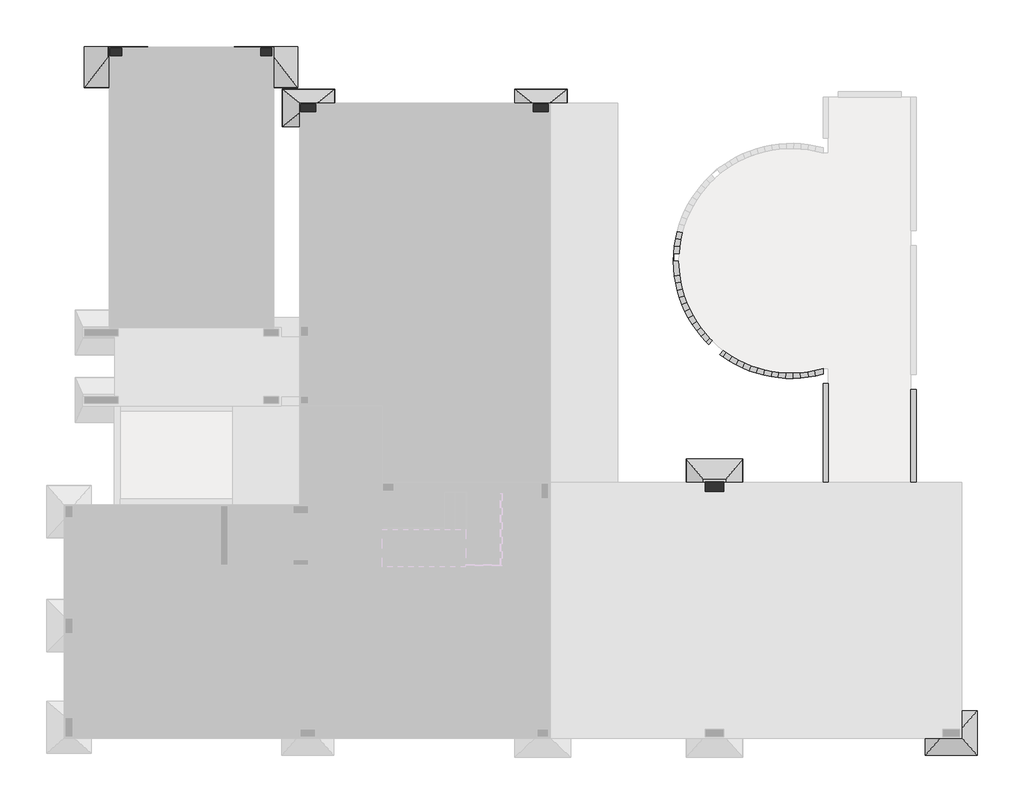
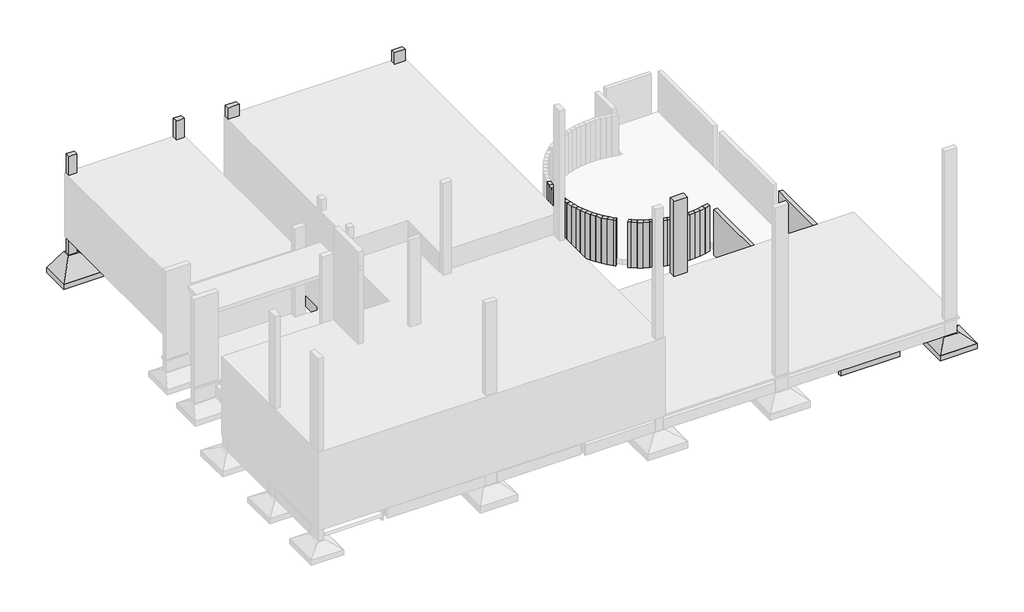
# One storey, part 3 of 4: 37 beams, 7 fasteners, 5 columns.
# Revit data of these elements (continued)
# Element 42 (IfcColumn, "TQS - Pilar retangular : 25.0 x 50.0") (continued)
#   SHA1 = "9F824B836982A58BF5E6376D71D0493ECBE449DE"
#   Revisão = ""
#   Tipo de carga = ""
#   Divisor de flexao = ""
#   Secao = "R 25/50 90°"
#   Configuracao = ""
#   Angulo (graus) = ""
#   Detalhamento = ""
#   Casos de vento manual = ""
#   Tipo = ""
#   Alcas = ""
#   Furos = ""
#   Pino = ""
#   Distribuicao = ""
#   Solidarizado = ""
#   Solidarizar na montagem = ""
#   Unir com o próximo = ""
#   Grupo pre moldado = ""
#   Verificado = ""
#   Concreto C = ""
#   Taxa de armadura (kgf/m³) = 0
#   Carga (tf/m²) = 0
#   Carga (tf/m) = 0
#   Carga (tf) = 0
#   Altura = 3.10 m
#   Rebaixo = 0.00 m
#   Altura da fundacao = 0.00 m
#   Largura = 0.00 m
#   Distancia a face = 0.00 m
#   Distancia ao eixo = 0.00 m
#   Resultado de Ensaios fck (MPa) = 0
#   Unique TQS ID = -31
#   Principal = yes
#   Nasce = yes
#   Morre = yes
#   Cabeca de Pilar = no
#   Structural Material = Concrete - Cast-in-Place Concrete
#   Phase Created = CC_AP/ESTR
#   Materials on its faces: "Concrete - Cast-in-Place Concrete"
# Element 43 (IfcFastener, "TQS - Sapata : S1")
#   Uso = "ESTRUTURA"
#   Titulo = "S1"
#   Chave = "-1407"
#   Tipo Elemento = "Fundação"
#   SHA1 = "D0614686ED5849A1EAB74F1A010678AA73C49ED4"
#   Revisão = ""
#   Tipo de carga = ""
#   Divisor de flexao = ""
#   Secao = ""
#   Configuracao = ""
#   Angulo (graus) = ""
#   Detalhamento = ""
#   Casos de vento manual = ""
#   Tipo = "Sapata"
#   Dimensoes = "110.0,170.0"
#   Estacas = ""
#   Calice = ""
#   Rugosidade = ""
#   Alcas = ""
#   Furos = ""
#   Pino = ""
#   Distribuicao = ""
#   Solidarizado = ""
#   Solidarizar na montagem = ""
#   Unir com o próximo = ""
#   Grupo pre moldado = ""
#   Verificado = ""
#   Concreto C = ""
#   Taxa de armadura (kgf/m³) = 0
#   Carga (tf/m²) = 0
#   Carga (tf/m) = 0
#   Carga (tf) = 0
#   Altura = 0.00 m
#   Rebaixo = 0.00 m
#   Pilar ficticio = 0.00 m
#   Topo = -0.10 m
#   Altura total = 0.60 m
#   Rodape = 0.00 m
#   Diametro = 0.00 m
#   Altura dentro do bloco = 0.00 m
#   Entre eixos = 0.00 m
#   Paredes = 0.00 m
#   Caimento = 0.00 m
#   Largura = 0.00 m
#   Distancia a face = 0.00 m
#   Distancia ao eixo = 0.00 m
#   Resultado de Ensaios fck (MPa) = 0
#   Unique TQS ID = -1407
#   Principal = yes
#   Phase Created = CC_AP/ESTR
#   Materials on its faces: "Concreto - Concreto concretado no local"
# Element 44 (IfcFastener, "TQS - Sapata : S12")
#   Uso = "ESTRUTURA"
#   Titulo = "S12"
#   Chave = "-1436"
#   Tipo Elemento = "Fundação"
#   SHA1 = "A28B53AB49304EFCBF9C768E884AA5FFCB5BBDAA"
#   Revisão = ""
#   Tipo de carga = ""
#   Divisor de flexao = ""
#   Secao = ""
#   Configuracao = ""
#   Angulo (graus) = ""
#   Detalhamento = ""
#   Casos de vento manual = ""
#   Tipo = "Sapata"
#   Dimensoes = "150.0,150.0"
#   Estacas = ""
#   Calice = ""
#   Rugosidade = ""
#   Alcas = ""
#   Furos = ""
#   Pino = ""
#   Distribuicao = ""
#   Solidarizado = ""
#   Solidarizar na montagem = ""
#   Unir com o próximo = ""
#   Grupo pre moldado = ""
#   Verificado = ""
#   Concreto C = ""
#   Taxa de armadura (kgf/m³) = 0
#   Carga (tf/m²) = 0
#   Carga (tf/m) = 0
#   Carga (tf) = 0
#   Altura = 0.00 m
#   Rebaixo = 0.00 m
#   Pilar ficticio = 0.00 m
#   Topo = -0.10 m
#   Altura total = 0.60 m
#   Rodape = 0.00 m
#   Diametro = 0.00 m
#   Altura dentro do bloco = 0.00 m
#   Entre eixos = 0.00 m
#   Paredes = 0.00 m
#   Caimento = 0.00 m
#   Largura = 0.00 m
#   Distancia a face = 0.00 m
#   Distancia ao eixo = 0.00 m
#   Resultado de Ensaios fck (MPa) = 0
#   Unique TQS ID = -1436
#   Principal = yes
#   Phase Created = CC_AP/ESTR
#   Materials on its faces: "Concreto - Concreto concretado no local"
# Element 45 (IfcFastener, "TQS - Sapata : S13")
#   Uso = "ESTRUTURA"
#   Titulo = "S13"
#   Chave = "-1457"
#   Tipo Elemento = "Fundação"
#   SHA1 = "BF7891B0F83325896F70E9D7259C0573D0C4C40D"
#   Revisão = ""
#   Tipo de carga = ""
#   Divisor de flexao = ""
#   Secao = ""
#   Configuracao = ""
#   Angulo (graus) = ""
#   Detalhamento = ""
#   Casos de vento manual = ""
#   Tipo = "Sapata"
#   Dimensoes = "150.0,150.0"
#   Estacas = ""
#   Calice = ""
#   Rugosidade = ""
#   Alcas = ""
#   Furos = ""
#   Pino = ""
#   Distribuicao = ""
#   Solidarizado = ""
#   Solidarizar na montagem = ""
#   Unir com o próximo = ""
#   Grupo pre moldado = ""
#   Verificado = ""
#   Concreto C = ""
#   Taxa de armadura (kgf/m³) = 0
#   Carga (tf/m²) = 0
#   Carga (tf/m) = 0
#   Carga (tf) = 0
#   Altura = 0.00 m
#   Rebaixo = 0.00 m
#   Pilar ficticio = 0.00 m
#   Topo = -0.10 m
#   Altura total = 0.50 m
#   Rodape = 0.00 m
#   Diametro = 0.00 m
#   Altura dentro do bloco = 0.00 m
#   Entre eixos = 0.00 m
#   Paredes = 0.00 m
#   Caimento = 0.00 m
#   Largura = 0.00 m
#   Distancia a face = 0.00 m
#   Distancia ao eixo = 0.00 m
#   Resultado de Ensaios fck (MPa) = 0
#   Unique TQS ID = -1457
#   Principal = yes
#   Phase Created = CC_AP/ESTR
#   Materials on its faces: "Concreto - Concreto concretado no local"
# Element 46 (IfcFastener, "TQS - Sapata : S2")
#   Uso = "ESTRUTURA"
#   Titulo = "S2"
#   Chave = "-1408"
#   Tipo Elemento = "Fundação"
#   SHA1 = "2282C10FF7FA64FC48FCFA0318D48FBC3A2ACDAC"
#   Revisão = ""
#   Tipo de carga = ""
#   Divisor de flexao = ""
#   Secao = ""
#   Configuracao = ""
#   Angulo (graus) = ""
#   Detalhamento = ""
#   Casos de vento manual = ""
#   Tipo = "Sapata"
#   Dimensoes = "110.0,170.0"
#   Estacas = ""
#   Calice = ""
#   Rugosidade = ""
#   Alcas = ""
#   Furos = ""
#   Pino = ""
#   Distribuicao = ""
#   Solidarizado = ""
#   Solidarizar na montagem = ""
#   Unir com o próximo = ""
#   Grupo pre moldado = ""
#   Verificado = ""
#   Concreto C = ""
#   Taxa de armadura (kgf/m³) = 0
#   Carga (tf/m²) = 0
#   Carga (tf/m) = 0
#   Carga (tf) = 0
#   Altura = 0.00 m
#   Rebaixo = 0.00 m
#   Pilar ficticio = 0.00 m
#   Topo = -0.10 m
#   Altura total = 0.60 m
#   Rodape = 0.00 m
#   Diametro = 0.00 m
#   Altura dentro do bloco = 0.00 m
#   Entre eixos = 0.00 m
#   Paredes = 0.00 m
#   Caimento = 0.00 m
#   Largura = 0.00 m
#   Distancia a face = 0.00 m
#   Distancia ao eixo = 0.00 m
#   Resultado de Ensaios fck (MPa) = 0
#   Unique TQS ID = -1408
#   Principal = yes
#   Phase Created = CC_AP/ESTR
#   Materials on its faces: "Concreto - Concreto concretado no local"
# Element 47 (IfcFastener, "TQS - Sapata : S24")
#   Uso = "ESTRUTURA"
#   Titulo = "S24"
#   Chave = "-1461"
#   Tipo Elemento = "Fundação"
#   SHA1 = "7859DB63F09D5F0F67BBBF72A3CA603880B25958"
#   Revisão = ""
#   Tipo de carga = ""
#   Divisor de flexao = ""
#   Secao = ""
#   Configuracao = ""
#   Angulo (graus) = ""
#   Detalhamento = ""
#   Casos de vento manual = ""
#   Tipo = "Sapata"
#   Dimensoes = "120.0,140.0"
#   Estacas = ""
#   Calice = ""
#   Rugosidade = ""
#   Alcas = ""
#   Furos = ""
#   Pino = ""
#   Distribuicao = ""
#   Solidarizado = ""
#   Solidarizar na montagem = ""
#   Unir com o próximo = ""
#   Grupo pre moldado = ""
#   Verificado = ""
#   Concreto C = ""
#   Taxa de armadura (kgf/m³) = 0
#   Carga (tf/m²) = 0
#   Carga (tf/m) = 0
#   Carga (tf) = 0
#   Altura = 0.00 m
#   Rebaixo = 0.00 m
#   Pilar ficticio = 0.00 m
#   Topo = -0.06 m
#   Altura total = 0.50 m
#   Rodape = 0.00 m
#   Diametro = 0.00 m
#   Altura dentro do bloco = 0.00 m
#   Entre eixos = 0.00 m
#   Paredes = 0.00 m
#   Caimento = 0.00 m
#   Largura = 0.00 m
#   Distancia a face = 0.00 m
#   Distancia ao eixo = 0.00 m
#   Resultado de Ensaios fck (MPa) = 0
#   Unique TQS ID = -1461
#   Principal = yes
#   Phase Created = CC_AP/ESTR
#   Materials on its faces: "Concreto - Concreto concretado no local"
# Element 48 (IfcFastener, "TQS - Sapata : S3")
#   Uso = "ESTRUTURA"
#   Titulo = "S3"
#   Chave = "-1405"
#   Tipo Elemento = "Fundação"
#   SHA1 = "E7F86A4529557F0178A31412CAAF120C6199F7FB"
#   Revisão = ""
#   Tipo de carga = ""
#   Divisor de flexao = ""
#   Secao = ""
#   Configuracao = ""
#   Angulo (graus) = ""
#   Detalhamento = ""
#   Casos de vento manual = ""
#   Tipo = "Sapata"
#   Dimensoes = "100.0,140.0"
#   Estacas = ""
#   Calice = ""
#   Rugosidade = ""
#   Alcas = ""
#   Furos = ""
#   Pino = ""
#   Distribuicao = ""
#   Solidarizado = ""
#   Solidarizar na montagem = ""
#   Unir com o próximo = ""
#   Grupo pre moldado = ""
#   Verificado = ""
#   Concreto C = ""
#   Taxa de armadura (kgf/m³) = 0
#   Carga (tf/m²) = 0
#   Carga (tf/m) = 0
#   Carga (tf) = 0
#   Altura = 0.00 m
#   Rebaixo = 0.00 m
#   Pilar ficticio = 0.00 m
#   Topo = 0.00 m
#   Altura total = 0.50 m
#   Rodape = 0.00 m
#   Diametro = 0.00 m
#   Altura dentro do bloco = 0.00 m
#   Entre eixos = 0.00 m
#   Paredes = 0.00 m
#   Caimento = 0.00 m
#   Largura = 0.00 m
#   Distancia a face = 0.00 m
#   Distancia ao eixo = 0.00 m
#   Resultado de Ensaios fck (MPa) = 0
#   Unique TQS ID = -1405
#   Principal = yes
#   Phase Created = CC_AP/ESTR
#   Materials on its faces: "Concreto - Concreto concretado no local"
# Element 49 (IfcFastener, "TQS - Sapata : S4")
#   Uso = "ESTRUTURA"
#   Titulo = "S4"
#   Chave = "-1406"
#   Tipo Elemento = "Fundação"
#   SHA1 = "1CBAC234F592DF4B85828C708D4D8DF50E3056D8"
#   Revisão = ""
#   Tipo de carga = ""
#   Divisor de flexao = ""
#   Secao = ""
#   Configuracao = ""
#   Angulo (graus) = ""
#   Detalhamento = ""
#   Casos de vento manual = ""
#   Tipo = "Sapata"
#   Dimensoes = "100.0,140.0"
#   Estacas = ""
#   Calice = ""
#   Rugosidade = ""
#   Alcas = ""
#   Furos = ""
#   Pino = ""
#   Distribuicao = ""
#   Solidarizado = ""
#   Solidarizar na montagem = ""
#   Unir com o próximo = ""
#   Grupo pre moldado = ""
#   Verificado = ""
#   Concreto C = ""
#   Taxa de armadura (kgf/m³) = 0
#   Carga (tf/m²) = 0
#   Carga (tf/m) = 0
#   Carga (tf) = 0
#   Altura = 0.00 m
#   Rebaixo = 0.00 m
#   Pilar ficticio = 0.00 m
#   Topo = 0.00 m
#   Altura total = 0.50 m
#   Rodape = 0.00 m
#   Diametro = 0.00 m
#   Altura dentro do bloco = 0.00 m
#   Entre eixos = 0.00 m
#   Paredes = 0.00 m
#   Caimento = 0.00 m
#   Largura = 0.00 m
#   Distancia a face = 0.00 m
#   Distancia ao eixo = 0.00 m
#   Resultado de Ensaios fck (MPa) = 0
#   Unique TQS ID = -1406
#   Principal = yes
#   Phase Created = CC_AP/ESTR
#   Materials on its faces: "Concreto - Concreto concretado no local"
# Materials
#   "Concrete - Cast-in-Place Concrete": class "Unassigned", colour RGB 192 192 192, transparency 0
#   "Concreto - Concreto concretado no local": class "Concreto", colour RGB 192 192 192, transparency 0
